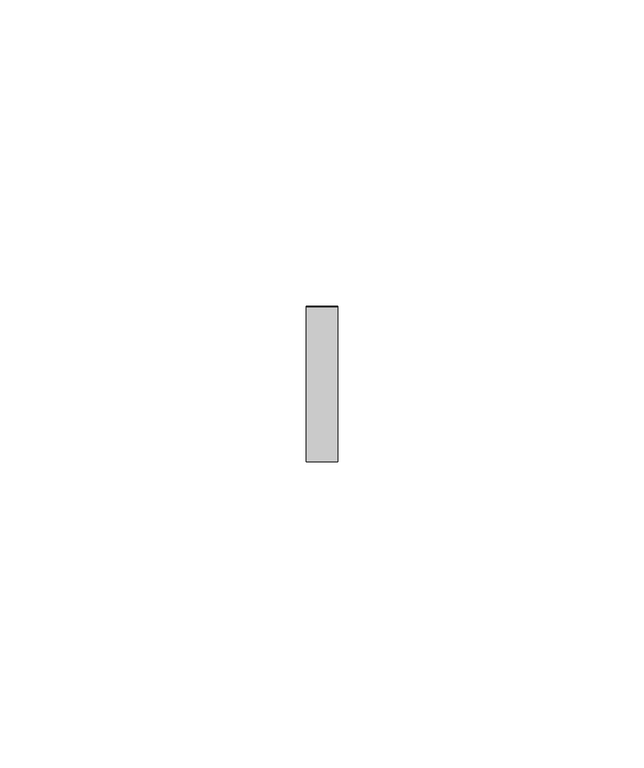
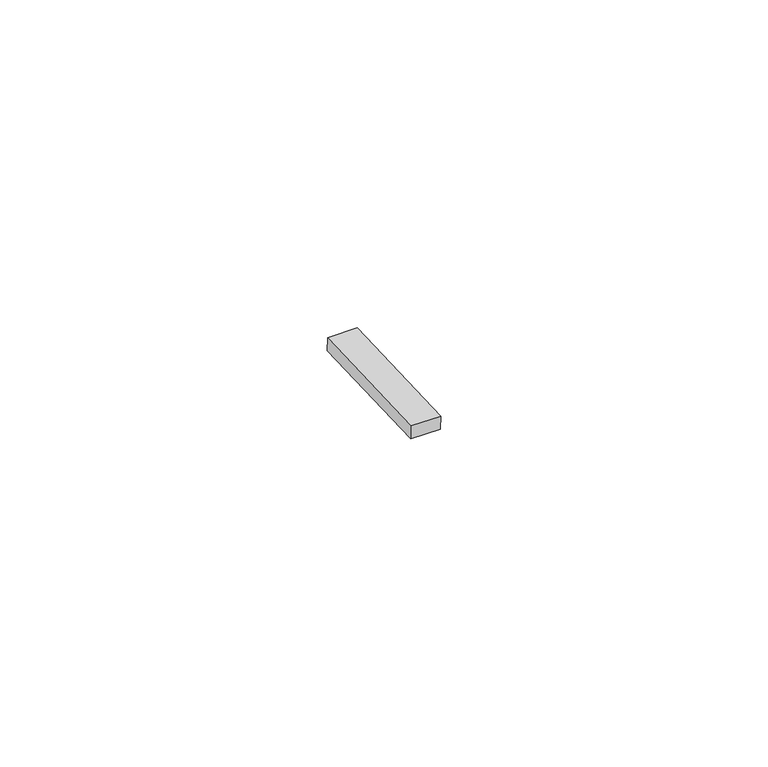
"""IFC4 building model written with IfcOpenShell, lengths in millimetres: proxy geometry, Inner panel:Inner panel:1:Inner panel:1 : Inner panel:Inner panel:300324:2:Inner panel:1:Inner panel:1 : Inner panel:Inner panel:300324:2 : Inner panel:Inner panel:1:Inner panel:1 : Inner panel:Inner panel:300324:300043:124 : Inner panel:Inner panel:1:Inner panel:1 : Inner panel:Inner panel:300324:2:Inner panel:1:Inner panel:1 : Inner panel:Inner panel:300324:2 : Inner panel:Inner panel:1:Inner panel:1 : Inner panel:Inner panel:300324:300043:308120."""

from ifc_helpers import new_model, si_unit, frame, origin, place, context, project, spatial, polyline, outline, extrude, source, transform, mapped, element, save


def generic_models_f918a1d4(model_context):
    return source(origin(), model_context, "Body", "SweptSolid", [
        extrude(outline(polyline([(0.0, -25.4), (0.0, 0.0), (5.2138089, 0.0), (5.2138089, -25.4), (0.0, -25.4)])), frame((592310.995117, -578253.2828061, 3981.0403755), z_axis=(0.0, -0.041630544712223896, 0.9991330730923502), x_axis=(-1.0, 0.0, 0.0)), (0.0, 0.0, 1.0), 2.4763745),
    ])


if __name__ == "__main__":
    model = new_model("IFC4")
    model_context = context("Model", 3, world=origin())
    ifc_project = project(units=[si_unit("LENGTHUNIT", "METRE", prefix="MILLI")], contexts=[model_context])
    site = spatial("IfcSite", under=ifc_project)
    building = spatial("IfcBuilding", under=site)
    placement = place(None, origin())
    generic_models_shape = generic_models_f918a1d4(model_context)
    element("IfcBuildingElementProxy", 1, Name="Inner panel:Inner panel:1:Inner panel:1 : Inner panel:Inner panel:300324:2:Inner panel:1:Inner panel:1 : Inner panel:Inner panel:300324:2 : Inner panel:Inner panel:1:Inner panel:1 : Inner panel:Inner panel:300324:300043:124 : Inner panel:Inner panel:1:Inner panel:1 : Inner panel:Inner panel:300324:2:Inner panel:1:Inner panel:1 : Inner panel:Inner panel:300324:2 : Inner panel:Inner panel:1:Inner panel:1 : Inner panel:Inner panel:300324:300043:308120", ObjectType="Inner panel:Inner panel:1:Inner panel:1 : Inner panel:Inner panel:300324:2:Inner panel:1:Inner panel:1 : Inner panel:Inner panel:300324:2 : Inner panel:Inner panel:1:Inner panel:1 : Inner panel:Inner panel:300324:300043:124 : Inner panel:Inner panel:1:Inner panel:1 : Inner panel:Inner panel:300324:2:Inner panel:1:Inner panel:1 : Inner panel:Inner panel:300324:2 : Inner panel:Inner panel:1:Inner panel:1 : Inner panel:Inner panel:300324:300043:308120", at=placement, inside=building, context=model_context, shape_type="MappedRepresentation", body=[
        mapped(generic_models_shape, transform((0.0, 0.0, 0.0), x_axis=(1.0, 0.0, 0.0), y_axis=(0.0, 1.0, 0.0), z_axis=(0.0, 0.0, 1.0))),
    ])
    save(model, "model.ifc")

# Revit data of these elements
# Type "Inner panel:Inner panel:1:Inner panel:1 : Inner panel:Inner panel:300324:2:Inner panel:1:Inner panel:1 : Inner panel:Inner panel:300324:2 : Inner panel:Inner panel:1:Inner panel:1 : Inner panel:Inner panel:300324:300043:124 : Inner panel:Inner panel:1:Inner panel:1 : Inner panel:Inner panel:300324:2:Inner panel:1:Inner panel:1 : Inner panel:Inner panel:300324:2 : Inner panel:Inner panel:1:Inner panel:1 : Inner panel:Inner panel:300324:300043:308120"
#   NameOverride = "Inner panel:Inner panel:1:Inner panel:1 : Inner panel:Inner panel:300324:2:Inner panel:1:Inner panel:1 : Inner panel:Inner panel:300324:2 : Inner panel:Inner panel:1:Inner panel:1 : Inner panel:Inner panel:300324:300043:308120"
#   ObjectTypeOverride = "Inner panel:1:Inner panel:1 : Inner panel:Inner panel:300324:2 : Inner panel:Inner panel:1:Inner panel:1 : Inner panel:Inner panel:300324:300043"
#   Reference = "Inner panel"
#   Tag = "308120"
# Element 1 (IfcBuildingElementProxy, "Inner panel:Inner panel:1:Inner panel:1 : Inner panel:Inner panel:300324:2:Inner panel:1:Inner panel:1 : Inner panel:Inner panel:300324:2 : Inner panel:Inner panel:1:Inner panel:1 : Inner panel:Inner panel:300324:300043:124 : Inner panel:Inner panel:1:Inner panel:1 : Inner panel:Inner panel:300324:2:Inner panel:1:Inner panel:1 : Inner panel:Inner panel:300324:2 : Inner panel:Inner panel:1:Inner panel:1 : Inner panel:Inner panel:300324:300043:308120")
#   Materials on its faces: "AT CLIP - 1\" WIDE NON ABSORBENT, WEATHER-RESISTANT NEOPRENE/EPDM/SBR FOAM"
# Materials
#   "AT CLIP - 1\" WIDE NON ABSORBENT, WEATHER-RESISTANT NEOPRENE/EPDM/SBR FOAM": class "Generic", colour RGB 85 85 85, transparency 0, Cost = 0
